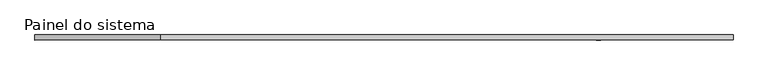
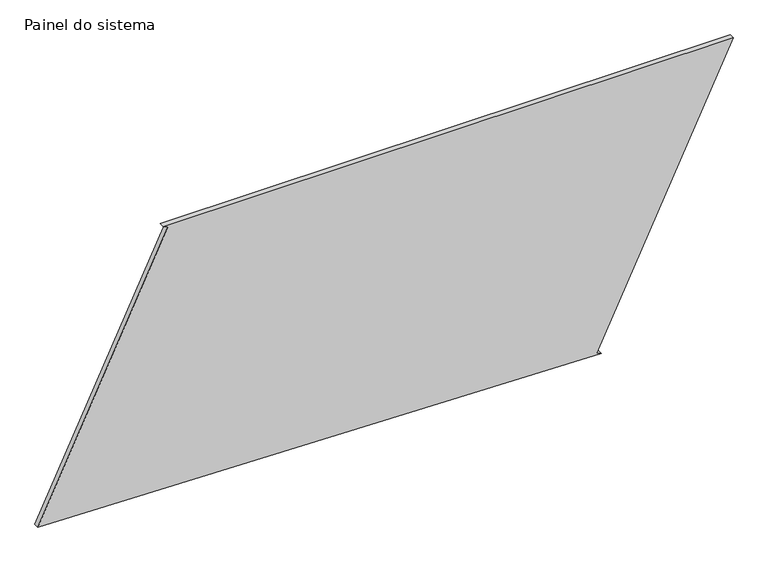
"""IFC4 building model written with IfcOpenShell, lengths in millimetres: plate geometry, Painel do sistema : Envidraçado."""

import ifcopenshell
import ifcopenshell.guid

model = None  # the IFC model being written
_history = None  # IfcOwnerHistory: only IFC2X3 demands one
_inside = {}  # id of a spatial element -> (the spatial element, [elements in it])
_under = {}  # id of a project, library or spatial element -> (it, [spatial elements below it])
_declared = {}  # id of a project -> (the project, [libraries it declares])
_typed = {}  # id of a type object -> (the type object, [elements of that type])
_made_of = {}  # id of a material, layer set ... -> (it, [elements and type objects made of it])


def new_model(schema):
    """Start an empty IFC model of exactly this schema.

    Asked for "IFC4X3", IfcOpenShell would pick the latest addendum, in which some entities
    have other attributes; the version numbers below select the first issue.
    IFC2X3 requires an IfcOwnerHistory on every rooted entity: one is made here for all.
    """
    global model, _history
    if schema == "IFC4X3":
        model = ifcopenshell.file(schema_version=(4, 3, 0, 0))
    else:
        model = ifcopenshell.file(schema=schema)
    _inside.clear()
    _under.clear()
    _declared.clear()
    _typed.clear()
    _made_of.clear()
    _history = None
    if model.schema == "IFC2X3":
        org = make("IfcOrganization", Name="unknown")
        user = make(
            "IfcPersonAndOrganization",
            ThePerson=make("IfcPerson", FamilyName="unknown"),
            TheOrganization=org,
        )
        app = make(
            "IfcApplication",
            ApplicationDeveloper=org,
            Version="unknown",
            ApplicationFullName="unknown",
            ApplicationIdentifier="unknown",
        )
        _history = make(
            "IfcOwnerHistory",
            OwningUser=user,
            OwningApplication=app,
            ChangeAction="ADDED",
            CreationDate=0,
        )
    return model


def make(cls, **values):
    """One entity of the class cls with the attributes given. An attribute that is None is left unset."""
    return model.create_entity(
        cls, **{name: value for name, value in values.items() if value is not None}
    )


def rooted(cls, **values):
    """An entity with a GlobalId (a new one), such as an element, a storey or a relation."""
    return make(cls, GlobalId=ifcopenshell.guid.new(), OwnerHistory=_history, **values)


def si_unit(unit_type, name, prefix=None):
    """IfcSIUnit, for example si_unit("LENGTHUNIT", "METRE", prefix="MILLI")."""
    return make("IfcSIUnit", UnitType=unit_type, Prefix=prefix, Name=name)


def assignment(units):
    """IfcUnitAssignment: the units of a project."""
    return None if units is None else make("IfcUnitAssignment", Units=units)


def point(xyz):
    """IfcCartesianPoint."""
    return None if xyz is None else make("IfcCartesianPoint", Coordinates=xyz)


def direction(xyz):
    """IfcDirection."""
    return None if xyz is None else make("IfcDirection", DirectionRatios=xyz)


def frame(location, z_axis=None, x_axis=None):
    """IfcAxis2Placement3D, a coordinate frame: its origin and axes. An axis left out is left unset."""
    return make(
        "IfcAxis2Placement3D",
        Location=point(location),
        Axis=direction(z_axis),
        RefDirection=direction(x_axis),
    )


def origin():
    """The frame at (0, 0, 0) with its axes left unset."""
    return frame((0.0, 0.0, 0.0))


def place(relative_to, where):
    """IfcLocalPlacement: puts the frame where relative to a parent placement (None: the world)."""
    return make(
        "IfcLocalPlacement", PlacementRelTo=relative_to, RelativePlacement=where
    )


def context(
    kind, dimensions, precision=None, world=None, true_north=None, identifier=None
):
    """IfcGeometricRepresentationContext, for example the 3D "Model" context."""
    return make(
        "IfcGeometricRepresentationContext",
        ContextIdentifier=identifier,
        ContextType=kind,
        CoordinateSpaceDimension=dimensions,
        Precision=precision,
        WorldCoordinateSystem=world,
        TrueNorth=true_north,
    )


def project(units=None, contexts=None):
    """IfcProject with its units and contexts."""
    return rooted(
        "IfcProject",
        Name="project",
        RepresentationContexts=contexts,
        UnitsInContext=assignment(units),
    )


def spatial(cls, under=None, at=None, **own):
    """A site, building, storey or space (cls), placed at a placement, below another one or the project."""
    s = rooted(cls, ObjectPlacement=at, **own)
    if under is not None:
        _under.setdefault(under.id(), (under, []))[1].append(s)
    return s


def polyline(points):
    """IfcPolyline through the points."""
    return make("IfcPolyline", Points=[point(p) for p in points])


def outline(outer, holes=None, kind="AREA"):
    """IfcArbitraryClosedProfileDef: a profile drawn as a closed curve; with holes, ...WithVoids."""
    if holes is None:
        return make("IfcArbitraryClosedProfileDef", ProfileType=kind, OuterCurve=outer)
    return make(
        "IfcArbitraryProfileDefWithVoids",
        ProfileType=kind,
        OuterCurve=outer,
        InnerCurves=holes,
    )


def extrude(swept, where, along, depth):
    """IfcExtrudedAreaSolid: the profile swept, set in the frame where, extruded along a direction by depth."""
    return make(
        "IfcExtrudedAreaSolid",
        SweptArea=swept,
        Position=where,
        ExtrudedDirection=direction(along),
        Depth=depth,
    )


def shape(context_of_items, identifier, shape_type, items):
    """IfcShapeRepresentation: the items that make up one representation, for example the "Body"."""
    return make(
        "IfcShapeRepresentation",
        ContextOfItems=context_of_items,
        RepresentationIdentifier=identifier,
        RepresentationType=shape_type,
        Items=items,
    )


def source(mapping_origin, context_of_items, identifier, shape_type, items):
    """IfcRepresentationMap: a shape defined once, which mapped items show again and again."""
    return make(
        "IfcRepresentationMap",
        MappingOrigin=mapping_origin,
        MappedRepresentation=shape(context_of_items, identifier, shape_type, items),
    )


def transform(
    local_origin,
    x_axis=None,
    y_axis=None,
    z_axis=None,
    scale=None,
    scale2=None,
    scale3=None,
    uniform=True,
):
    """IfcCartesianTransformationOperator3D, or its non-uniform kind. x_axis, y_axis, z_axis: its Axis1, 2, 3."""
    if uniform:
        return make(
            "IfcCartesianTransformationOperator3D",
            Axis1=direction(x_axis),
            Axis2=direction(y_axis),
            LocalOrigin=point(local_origin),
            Scale=scale,
            Axis3=direction(z_axis),
        )
    return make(
        "IfcCartesianTransformationOperator3DnonUniform",
        Axis1=direction(x_axis),
        Axis2=direction(y_axis),
        LocalOrigin=point(local_origin),
        Scale=scale,
        Axis3=direction(z_axis),
        Scale2=scale2,
        Scale3=scale3,
    )


def mapped(mapping_source, mapping_target):
    """IfcMappedItem: shows the shape of a source again, moved by a transform."""
    return make(
        "IfcMappedItem", MappingSource=mapping_source, MappingTarget=mapping_target
    )


def made_of(thing, what):
    """Note that an element or type object is made of a material, layer set ...; save() writes the relation."""
    if what is not None:
        _made_of.setdefault(what.id(), (what, []))[1].append(thing)
    return thing


def element(
    cls,
    number,
    at=None,
    inside=None,
    cuts=None,
    type_object=None,
    material=None,
    context=None,
    identifier="Body",
    shape_type=None,
    held_by="IfcProductDefinitionShape",
    body=None,
    shapes=None,
    **own,
):
    """One element of the class cls, such as IfcWall. Its Tag is "e" and its number.

    at: its placement. inside: the storey or other place that contains it. cuts: it is an
    opening in that element (IfcRelVoidsElement). A single representation is given by context,
    identifier, shape_type and body (its items); several are given by shapes. held_by: the class
    of the entity that holds the representations. save() writes the other relations.
    """
    e = rooted(cls, Tag="e%d" % number, ObjectPlacement=at, **own)
    if body is not None:
        shapes = [shape(context, identifier, shape_type, body)]
    if shapes is not None:
        e.Representation = make(held_by, Representations=shapes)
    if inside is not None:
        _inside.setdefault(inside.id(), (inside, []))[1].append(e)
    if cuts is not None:
        rooted(
            "IfcRelVoidsElement", RelatingBuildingElement=cuts, RelatedOpeningElement=e
        )
    if type_object is not None:
        _typed.setdefault(type_object.id(), (type_object, []))[1].append(e)
    return made_of(e, material)


def aggregate(whole, parts):
    """IfcRelAggregates: a whole, such as a stair, and the parts it consists of."""
    return rooted("IfcRelAggregates", RelatingObject=whole, RelatedObjects=parts)


def save(model, path):
    """Write the relations noted so far, then the file.

    IfcRelAggregates (storeys below a building ...), IfcRelContainedInSpatialStructure (elements
    in a storey), IfcRelDefinesByType, IfcRelAssociatesMaterial and IfcRelDeclares: one each for
    every whole, place, type object, material and project.
    """
    for whole, parts in _under.values():
        aggregate(whole, parts)
    for where, things in _inside.values():
        rooted(
            "IfcRelContainedInSpatialStructure",
            RelatedElements=things,
            RelatingStructure=where,
        )
    for kind, things in _typed.values():
        rooted("IfcRelDefinesByType", RelatedObjects=things, RelatingType=kind)
    for what, things in _made_of.values():
        rooted("IfcRelAssociatesMaterial", RelatedObjects=things, RelatingMaterial=what)
    for by, libraries in _declared.values():
        rooted("IfcRelDeclares", RelatingContext=by, RelatedDefinitions=libraries)
    model.write(path)


def painel_do_sistema_f90cb54f(model_context):
    return source(origin(), model_context, "Body", "SweptSolid", [
        extrude(outline(polyline([(0.0, 1069.0381366), (10.7698497, 1046.4768792), (1426.4417808, 1722.2625214), (1426.4417808, -1100.7504936), (1415.6719311, -1078.1892361), (66.4327426, -1722.2625214), (0.0, 1069.0381366)])), frame((0.0, 24.5, 0.0), z_axis=(0.0, 1.0, 0.0), x_axis=(0.0, 0.0, 1.0)), (0.0, 0.0, 1.0), 25.0),
    ])


if __name__ == "__main__":
    model = new_model("IFC4")
    model_context = context("Model", 3, world=origin())
    ifc_project = project(units=[si_unit("LENGTHUNIT", "METRE", prefix="MILLI")], contexts=[model_context])
    site = spatial("IfcSite", under=ifc_project)
    building = spatial("IfcBuilding", under=site)
    placement = place(None, origin())
    painel_do_sistema_shape = painel_do_sistema_f90cb54f(model_context)
    element("IfcPlate", 1, ObjectType="Painel do sistema : Envidraçado", at=placement, inside=building, context=model_context, shape_type="MappedRepresentation", body=[
        mapped(painel_do_sistema_shape, transform((0.0, 0.0, 0.0), x_axis=(1.0, 0.0, 0.0), y_axis=(0.0, 1.0, 0.0), z_axis=(0.0, 0.0, 1.0))),
    ])
    save(model, "model.ifc")

# Revit data of these elements
# Type "Painel do sistema : Envidraçado"
#   Construction Type Id = "GSP4R"
#   Analytic Construction = "Vidraça única Pilkington 1/8 pol"
#   Visual Light Transmittance = 0.9
#   Solar Heat Gain Coefficient = 0.86
#   Heat Transfer Coefficient (U) = 6.7069 W/(m²·K)
# Element 1 (IfcPlate, "Painel do sistema : Envidraçado")
#   Materials on its faces: "Vidro"
# Materials
#   "Vidro": class "Vidro", colour RGB 0 128 192, transparency 0.9, Description = "Vidro de sílica", Cost = 0
